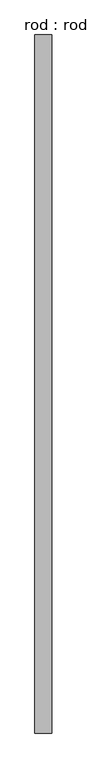
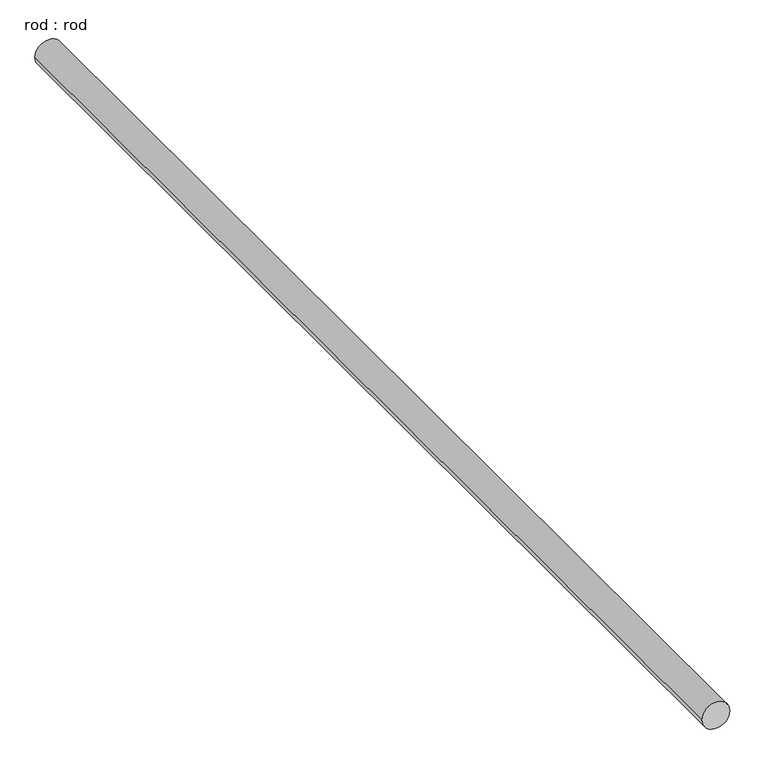
"""IFC4 building model written with IfcOpenShell, lengths in millimetres: proxy geometry, rod : rod."""

from ifc_helpers import new_model, si_unit, point, frame, frame_2d, origin, place, context, project, spatial, circle_curve, trimmed, segment, composite_curve, outline, extrude, source, transform, mapped, element, save


def rod_rod_68992995(model_context):
    return source(origin(), model_context, "Body", "SweptSolid", [
        extrude(outline(composite_curve([segment(trimmed(circle_curve(frame_2d((0.0108462, 0.0)), 200.0), [point((0.0108462, 200.0))], [point((0.0108462, -200.0))], False, "CARTESIAN"), True, "CONTINUOUS"), segment(trimmed(circle_curve(frame_2d((0.0108462, 0.0)), 200.0), [point((0.0108462, -200.0))], [point((0.0108462, 200.0))], False, "CARTESIAN"), True, "CONTINUOUS")], self_intersect=False)), frame((0.0, -4197.4499561, 0.0), z_axis=(0.0, 1.0, 0.0), x_axis=(0.0, 0.0, 1.0)), (0.0, 0.0, 1.0), 16580.3571429),
    ])


if __name__ == "__main__":
    model = new_model("IFC4")
    model_context = context("Model", 3, world=origin())
    ifc_project = project(units=[si_unit("LENGTHUNIT", "METRE", prefix="MILLI")], contexts=[model_context])
    site = spatial("IfcSite", under=ifc_project)
    building = spatial("IfcBuilding", under=site)
    placement = place(None, origin())
    rod_rod_shape = rod_rod_68992995(model_context)
    element("IfcBuildingElementProxy", 1, Name="rod : rod", ObjectType="rod : rod", at=placement, inside=building, context=model_context, shape_type="MappedRepresentation", body=[
        mapped(rod_rod_shape, transform((0.0, 0.0, 0.0), x_axis=(1.0, 0.0, 0.0), y_axis=(0.0, 1.0, 0.0), z_axis=(0.0, 0.0, 1.0))),
    ])
    save(model, "model.ifc")

# Revit data of these elements
# Type "rod : rod"
#   Default Elevation = 0
